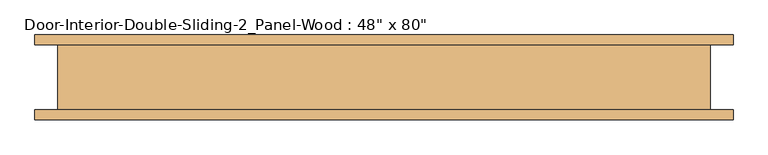
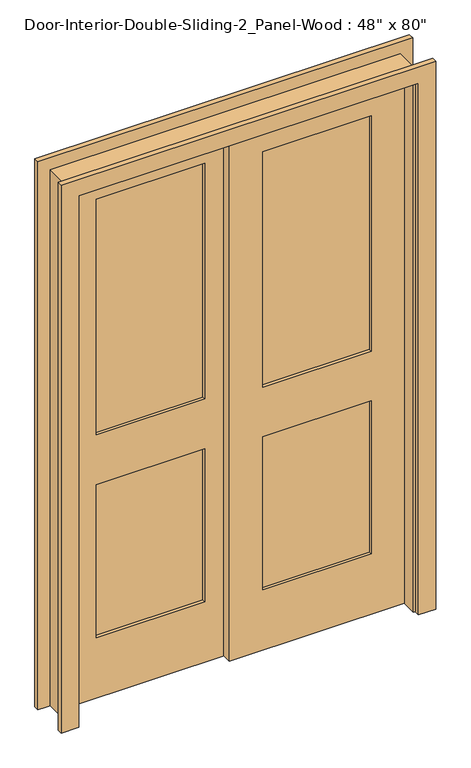
"""IFC4 building model written with IfcOpenShell, lengths in millimetres: door geometry."""

import ifcopenshell
import ifcopenshell.guid

model = None  # the IFC model being written
_history = None  # IfcOwnerHistory: only IFC2X3 demands one
_inside = {}  # id of a spatial element -> (the spatial element, [elements in it])
_under = {}  # id of a project, library or spatial element -> (it, [spatial elements below it])
_declared = {}  # id of a project -> (the project, [libraries it declares])
_typed = {}  # id of a type object -> (the type object, [elements of that type])
_made_of = {}  # id of a material, layer set ... -> (it, [elements and type objects made of it])


def new_model(schema):
    """Start an empty IFC model of exactly this schema.

    Asked for "IFC4X3", IfcOpenShell would pick the latest addendum, in which some entities
    have other attributes; the version numbers below select the first issue.
    IFC2X3 requires an IfcOwnerHistory on every rooted entity: one is made here for all.
    """
    global model, _history
    if schema == "IFC4X3":
        model = ifcopenshell.file(schema_version=(4, 3, 0, 0))
    else:
        model = ifcopenshell.file(schema=schema)
    _inside.clear()
    _under.clear()
    _declared.clear()
    _typed.clear()
    _made_of.clear()
    _history = None
    if model.schema == "IFC2X3":
        org = make("IfcOrganization", Name="unknown")
        user = make(
            "IfcPersonAndOrganization",
            ThePerson=make("IfcPerson", FamilyName="unknown"),
            TheOrganization=org,
        )
        app = make(
            "IfcApplication",
            ApplicationDeveloper=org,
            Version="unknown",
            ApplicationFullName="unknown",
            ApplicationIdentifier="unknown",
        )
        _history = make(
            "IfcOwnerHistory",
            OwningUser=user,
            OwningApplication=app,
            ChangeAction="ADDED",
            CreationDate=0,
        )
    return model


def make(cls, **values):
    """One entity of the class cls with the attributes given. An attribute that is None is left unset."""
    return model.create_entity(
        cls, **{name: value for name, value in values.items() if value is not None}
    )


def rooted(cls, **values):
    """An entity with a GlobalId (a new one), such as an element, a storey or a relation."""
    return make(cls, GlobalId=ifcopenshell.guid.new(), OwnerHistory=_history, **values)


def si_unit(unit_type, name, prefix=None):
    """IfcSIUnit, for example si_unit("LENGTHUNIT", "METRE", prefix="MILLI")."""
    return make("IfcSIUnit", UnitType=unit_type, Prefix=prefix, Name=name)


def assignment(units):
    """IfcUnitAssignment: the units of a project."""
    return None if units is None else make("IfcUnitAssignment", Units=units)


def point(xyz):
    """IfcCartesianPoint."""
    return None if xyz is None else make("IfcCartesianPoint", Coordinates=xyz)


def direction(xyz):
    """IfcDirection."""
    return None if xyz is None else make("IfcDirection", DirectionRatios=xyz)


def frame(location, z_axis=None, x_axis=None):
    """IfcAxis2Placement3D, a coordinate frame: its origin and axes. An axis left out is left unset."""
    return make(
        "IfcAxis2Placement3D",
        Location=point(location),
        Axis=direction(z_axis),
        RefDirection=direction(x_axis),
    )


def origin():
    """The frame at (0, 0, 0) with its axes left unset."""
    return frame((0.0, 0.0, 0.0))


def place(relative_to, where):
    """IfcLocalPlacement: puts the frame where relative to a parent placement (None: the world)."""
    return make(
        "IfcLocalPlacement", PlacementRelTo=relative_to, RelativePlacement=where
    )


def context(
    kind, dimensions, precision=None, world=None, true_north=None, identifier=None
):
    """IfcGeometricRepresentationContext, for example the 3D "Model" context."""
    return make(
        "IfcGeometricRepresentationContext",
        ContextIdentifier=identifier,
        ContextType=kind,
        CoordinateSpaceDimension=dimensions,
        Precision=precision,
        WorldCoordinateSystem=world,
        TrueNorth=true_north,
    )


def project(units=None, contexts=None):
    """IfcProject with its units and contexts."""
    return rooted(
        "IfcProject",
        Name="project",
        RepresentationContexts=contexts,
        UnitsInContext=assignment(units),
    )


def spatial(cls, under=None, at=None, **own):
    """A site, building, storey or space (cls), placed at a placement, below another one or the project."""
    s = rooted(cls, ObjectPlacement=at, **own)
    if under is not None:
        _under.setdefault(under.id(), (under, []))[1].append(s)
    return s


def polyline(points):
    """IfcPolyline through the points."""
    return make("IfcPolyline", Points=[point(p) for p in points])


def outline(outer, holes=None, kind="AREA"):
    """IfcArbitraryClosedProfileDef: a profile drawn as a closed curve; with holes, ...WithVoids."""
    if holes is None:
        return make("IfcArbitraryClosedProfileDef", ProfileType=kind, OuterCurve=outer)
    return make(
        "IfcArbitraryProfileDefWithVoids",
        ProfileType=kind,
        OuterCurve=outer,
        InnerCurves=holes,
    )


def extrude(swept, where, along, depth):
    """IfcExtrudedAreaSolid: the profile swept, set in the frame where, extruded along a direction by depth."""
    return make(
        "IfcExtrudedAreaSolid",
        SweptArea=swept,
        Position=where,
        ExtrudedDirection=direction(along),
        Depth=depth,
    )


def shape(context_of_items, identifier, shape_type, items):
    """IfcShapeRepresentation: the items that make up one representation, for example the "Body"."""
    return make(
        "IfcShapeRepresentation",
        ContextOfItems=context_of_items,
        RepresentationIdentifier=identifier,
        RepresentationType=shape_type,
        Items=items,
    )


def source(mapping_origin, context_of_items, identifier, shape_type, items):
    """IfcRepresentationMap: a shape defined once, which mapped items show again and again."""
    return make(
        "IfcRepresentationMap",
        MappingOrigin=mapping_origin,
        MappedRepresentation=shape(context_of_items, identifier, shape_type, items),
    )


def transform(
    local_origin,
    x_axis=None,
    y_axis=None,
    z_axis=None,
    scale=None,
    scale2=None,
    scale3=None,
    uniform=True,
):
    """IfcCartesianTransformationOperator3D, or its non-uniform kind. x_axis, y_axis, z_axis: its Axis1, 2, 3."""
    if uniform:
        return make(
            "IfcCartesianTransformationOperator3D",
            Axis1=direction(x_axis),
            Axis2=direction(y_axis),
            LocalOrigin=point(local_origin),
            Scale=scale,
            Axis3=direction(z_axis),
        )
    return make(
        "IfcCartesianTransformationOperator3DnonUniform",
        Axis1=direction(x_axis),
        Axis2=direction(y_axis),
        LocalOrigin=point(local_origin),
        Scale=scale,
        Axis3=direction(z_axis),
        Scale2=scale2,
        Scale3=scale3,
    )


def mapped(mapping_source, mapping_target):
    """IfcMappedItem: shows the shape of a source again, moved by a transform."""
    return make(
        "IfcMappedItem", MappingSource=mapping_source, MappingTarget=mapping_target
    )


def made_of(thing, what):
    """Note that an element or type object is made of a material, layer set ...; save() writes the relation."""
    if what is not None:
        _made_of.setdefault(what.id(), (what, []))[1].append(thing)
    return thing


def element(
    cls,
    number,
    at=None,
    inside=None,
    cuts=None,
    type_object=None,
    material=None,
    context=None,
    identifier="Body",
    shape_type=None,
    held_by="IfcProductDefinitionShape",
    body=None,
    shapes=None,
    **own,
):
    """One element of the class cls, such as IfcWall. Its Tag is "e" and its number.

    at: its placement. inside: the storey or other place that contains it. cuts: it is an
    opening in that element (IfcRelVoidsElement). A single representation is given by context,
    identifier, shape_type and body (its items); several are given by shapes. held_by: the class
    of the entity that holds the representations. save() writes the other relations.
    """
    e = rooted(cls, Tag="e%d" % number, ObjectPlacement=at, **own)
    if body is not None:
        shapes = [shape(context, identifier, shape_type, body)]
    if shapes is not None:
        e.Representation = make(held_by, Representations=shapes)
    if inside is not None:
        _inside.setdefault(inside.id(), (inside, []))[1].append(e)
    if cuts is not None:
        rooted(
            "IfcRelVoidsElement", RelatingBuildingElement=cuts, RelatedOpeningElement=e
        )
    if type_object is not None:
        _typed.setdefault(type_object.id(), (type_object, []))[1].append(e)
    return made_of(e, material)


def aggregate(whole, parts):
    """IfcRelAggregates: a whole, such as a stair, and the parts it consists of."""
    return rooted("IfcRelAggregates", RelatingObject=whole, RelatedObjects=parts)


def save(model, path):
    """Write the relations noted so far, then the file.

    IfcRelAggregates (storeys below a building ...), IfcRelContainedInSpatialStructure (elements
    in a storey), IfcRelDefinesByType, IfcRelAssociatesMaterial and IfcRelDeclares: one each for
    every whole, place, type object, material and project.
    """
    for whole, parts in _under.values():
        aggregate(whole, parts)
    for where, things in _inside.values():
        rooted(
            "IfcRelContainedInSpatialStructure",
            RelatedElements=things,
            RelatingStructure=where,
        )
    for kind, things in _typed.values():
        rooted("IfcRelDefinesByType", RelatedObjects=things, RelatingType=kind)
    for what, things in _made_of.values():
        rooted("IfcRelAssociatesMaterial", RelatedObjects=things, RelatingMaterial=what)
    for by, libraries in _declared.values():
        rooted("IfcRelDeclares", RelatingContext=by, RelatedDefinitions=libraries)
    model.write(path)


def door_f5052075(model_context):
    return source(origin(), model_context, "Body", "SweptSolid", [
        extrude(outline(polyline([(488.95, 2.1166667), (95.25, 2.1166667), (95.25, 13.7583333), (488.95, 13.7583333), (488.95, 2.1166667)])), frame((0.0, 0.0, 1009.65), z_axis=(0.0, 0.0, 1.0), x_axis=(1.0, 0.0, 0.0)), (0.0, 0.0, 1.0), 903.2875),
        extrude(outline(polyline([(488.95, 2.1166667), (95.25, 2.1166667), (95.25, 13.7583333), (488.95, 13.7583333), (488.95, 2.1166667)])), frame((0.0, 0.0, 231.775), z_axis=(0.0, 0.0, 1.0), x_axis=(1.0, 0.0, 0.0)), (0.0, 0.0, 1.0), 587.375),
        extrude(outline(polyline([(2032.0, -25.4), (0.0, -25.4), (0.0, 609.6), (2032.0, 609.6), (2032.0, -25.4)]), holes=[polyline([(1912.9375, 95.25), (1912.9375, 488.95), (1009.65, 488.95), (1009.65, 95.25), (1912.9375, 95.25)]), polyline([(819.15, 95.25), (819.15, 488.95), (231.775, 488.95), (231.775, 95.25), (819.15, 95.25)])]), frame((0.0, -9.525, 0.0), z_axis=(0.0, 1.0, 0.0), x_axis=(0.0, 0.0, 1.0)), (0.0, 0.0, 1.0), 34.925),
        extrude(outline(polyline([(-95.25, 37.0416667), (-488.95, 37.0416667), (-488.95, 48.6833333), (-95.25, 48.6833333), (-95.25, 37.0416667)])), frame((0.0, 0.0, 1009.65), z_axis=(0.0, 0.0, 1.0), x_axis=(1.0, 0.0, 0.0)), (0.0, 0.0, 1.0), 903.2875),
        extrude(outline(polyline([(-95.25, 37.0416667), (-488.95, 37.0416667), (-488.95, 48.6833333), (-95.25, 48.6833333), (-95.25, 37.0416667)])), frame((0.0, 0.0, 231.775), z_axis=(0.0, 0.0, 1.0), x_axis=(1.0, 0.0, 0.0)), (0.0, 0.0, 1.0), 587.375),
        extrude(outline(polyline([(2032.0, -609.6), (0.0, -609.6), (0.0, 25.4), (2032.0, 25.4), (2032.0, -609.6)]), holes=[polyline([(1912.9375, -488.95), (1912.9375, -95.25), (1009.65, -95.25), (1009.65, -488.95), (1912.9375, -488.95)]), polyline([(819.15, -488.95), (819.15, -95.25), (231.775, -95.25), (231.775, -488.95), (819.15, -488.95)])]), frame((0.0, 25.4, 0.0), z_axis=(0.0, 1.0, 0.0), x_axis=(0.0, 0.0, 1.0)), (0.0, 0.0, 1.0), 34.925),
        extrude(outline(polyline([(0.0, 609.6), (0.0, 635.0), (2057.4, 635.0), (2057.4, -635.0), (0.0, -635.0), (0.0, -609.6), (2032.0, -609.6), (2032.0, 609.6), (0.0, 609.6)])), frame((0.0, -66.675, 0.0), z_axis=(0.0, 1.0, 0.0), x_axis=(0.0, 0.0, 1.0)), (0.0, 0.0, 1.0), 127.0),
        extrude(outline(polyline([(0.0, 615.95), (0.0, 679.45), (2101.85, 679.45), (2101.85, -679.45), (0.0, -679.45), (0.0, -615.95), (2038.35, -615.95), (2038.35, 615.95), (0.0, 615.95)])), frame((0.0, -85.725, 0.0), z_axis=(0.0, 1.0, 0.0), x_axis=(0.0, 0.0, 1.0)), (0.0, 0.0, 1.0), 19.05),
        extrude(outline(polyline([(0.0, 615.95), (0.0, 679.45), (2101.85, 679.45), (2101.85, -679.45), (0.0, -679.45), (0.0, -615.95), (2038.35, -615.95), (2038.35, 615.95), (0.0, 615.95)])), frame((0.0, 60.325, 0.0), z_axis=(0.0, 1.0, 0.0), x_axis=(0.0, 0.0, 1.0)), (0.0, 0.0, 1.0), 19.05),
    ])


if __name__ == "__main__":
    model = new_model("IFC4")
    model_context = context("Model", 3, world=origin())
    ifc_project = project(units=[si_unit("LENGTHUNIT", "METRE", prefix="MILLI")], contexts=[model_context])
    site = spatial("IfcSite", under=ifc_project)
    building = spatial("IfcBuilding", under=site)
    placement = place(None, origin())
    door_shape = door_f5052075(model_context)
    element("IfcDoor", 1, ObjectType="Door-Interior-Double-Sliding-2_Panel-Wood : 48\" x 80\"", at=placement, inside=building, context=model_context, shape_type="MappedRepresentation", body=[
        mapped(door_shape, transform((0.0, 0.0, 0.0), x_axis=(1.0, 0.0, 0.0), y_axis=(0.0, 1.0, 0.0), z_axis=(0.0, 0.0, 1.0))),
    ])
    save(model, "model.ifc")

# Revit data of these elements
# Type "Door-Interior-Double-Sliding-2_Panel-Wood : 48\" x 80\""
#   Type Mark = "22"
#   Assembly Code = "C1020300"
#   Analytic Construction = "Wooden"
#   Top Rail = 0' - 4 11/16"
#   Thickness = 0' - 1 3/8"
#   Thermal Resistance (R) = 2.5876 (h·ft²·°F)/BTU
#   Stiles = 0' - 4 3/4"
#   Rough Width = 4' - 2"
#   Rough Height = 6' - 9"
#   Lock Rail = 0' - 7 1/2"
#   Height = 6' - 8"
#   Width = 4' - 0"
#   Heat Transfer Coefficient (U) = 0.3865 BTU/(h·ft²·°F)
#   Bottom Rail = 0' - 9 1/8"
#   Trim Material = Cherry
#   Panel Material = Cherry
#   Frame Material = Cherry
#   Visual Light Transmittance = 0
#   Solar Heat Gain Coefficient = 0
#   Wall Closure = (empty or 0)
#   Function = (empty or 0)
# Element 1 (IfcDoor, "Door-Interior-Double-Sliding-2_Panel-Wood : 48\" x 80\"")
#   Materials on its faces: "Cherry"
# Materials
#   "Cherry": class "Wood", colour RGB 226 177 128, transparency 0, Description = "Prunus Serotina", Cost = 0
